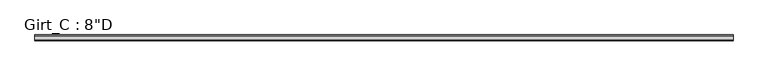
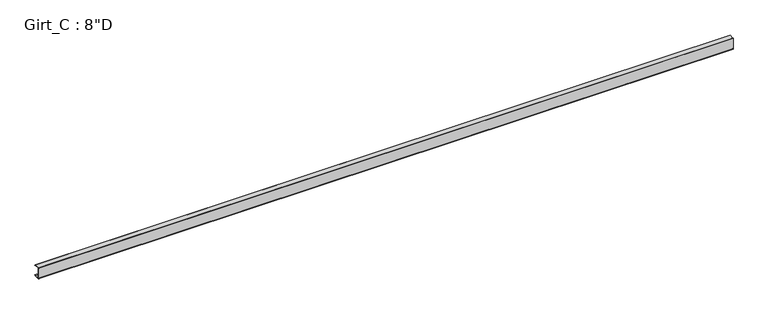
"""IFC4 building model written with IfcOpenShell, lengths in millimetres: beam geometry."""

from ifc_helpers import new_model, si_unit, point, frame, frame_2d, origin, place, context, project, spatial, polyline, circle_curve, trimmed, segment, composite_curve, outline, extrude, source, transform, mapped, element, save


def beam_da26f20a(model_context):
    return source(origin(), model_context, "Body", "SweptSolid", [
        extrude(outline(composite_curve([segment(polyline([(87.5109375, 101.6), (99.7560415, 87.0068534), (97.6278742, 85.221109), (86.2154765, 98.821875), (3.3005807, 98.821875)]), True, "CONTINUOUS"), segment(trimmed(circle_curve(frame_2d((3.3741066, 96.8381931)), 1.9850441), [point((3.3005807, 98.821875))], [point((1.3890625, 96.8381931))], True, "CARTESIAN"), True, "CONTINUOUS"), segment(polyline([(1.3890625, 96.8381931), (1.3890625, -96.8389339)]), True, "CONTINUOUS"), segment(trimmed(circle_curve(frame_2d((3.3748024, -96.8389339)), 1.9857399), [point((1.3890625, -96.8389339))], [point((3.2694106, -98.821875))], True, "CARTESIAN"), True, "CONTINUOUS"), segment(polyline([(3.2694106, -98.821875), (86.2154765, -98.821875), (97.6510975, -85.1934327), (99.7792647, -86.979177), (87.5109375, -101.6), (3.3734375, -101.6)]), True, "CONTINUOUS"), segment(trimmed(circle_curve(frame_2d((3.3734375, -96.8375)), 4.7625), [point((3.3734375, -101.6))], [point((-1.3890625, -96.8375))], False, "CARTESIAN"), True, "CONTINUOUS"), segment(polyline([(-1.3890625, -96.8375), (-1.3890625, 96.8375)]), True, "CONTINUOUS"), segment(trimmed(circle_curve(frame_2d((3.3734375, 96.8375)), 4.7625), [point((-1.3890625, 96.8375))], [point((3.3734375, 101.6))], False, "CARTESIAN"), True, "CONTINUOUS"), segment(polyline([(3.3734375, 101.6), (87.5109375, 101.6)]), True, "CONTINUOUS")], self_intersect=False)), frame((-6000.75, 0.0, 0.0), z_axis=(1.0, 0.0, 0.0), x_axis=(0.0, 1.0, 0.0)), (0.0, 0.0, 1.0), 12217.4),
    ])


if __name__ == "__main__":
    model = new_model("IFC4")
    model_context = context("Model", 3, world=origin())
    ifc_project = project(units=[si_unit("LENGTHUNIT", "METRE", prefix="MILLI")], contexts=[model_context])
    site = spatial("IfcSite", under=ifc_project)
    building = spatial("IfcBuilding", under=site)
    placement = place(None, origin())
    beam_shape = beam_da26f20a(model_context)
    element("IfcBeam", 1, ObjectType="Girt_C : 8\"D", at=placement, inside=building, context=model_context, shape_type="MappedRepresentation", body=[
        mapped(beam_shape, transform((0.0, 0.0, 0.0), x_axis=(1.0, 0.0, 0.0), y_axis=(0.0, 1.0, 0.0), z_axis=(0.0, 0.0, 1.0))),
    ])
    save(model, "model.ifc")

# Revit data of these elements
# Type "Girt_C : 8\"D"
#   half leg = 0' - 1 3/4"
#   Web_Thickness = 0' - 0 7/64"
#   Length [instance default] = 10' - 0"
#   Leg_1 = 0' - 3 1/2"
#   Height = 0' - 8"
#   Structural Material [instance default] = none
# Element 1 (IfcBeam, "Girt_C : 8\"D")
#   Structural Material = CEE' SECTION (8.0x3.5C - SEE STRUCT. DWGS)
#   Materials on its faces: "CEE' SECTION (8.0x3.5C - SEE STRUCT. DWGS)"
# Materials
#   "CEE' SECTION (8.0x3.5C - SEE STRUCT. DWGS)": class "Metal", colour RGB 137 146 153, transparency 0, Description = "Steel, mill finish", Cost = 0
